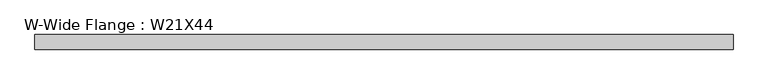
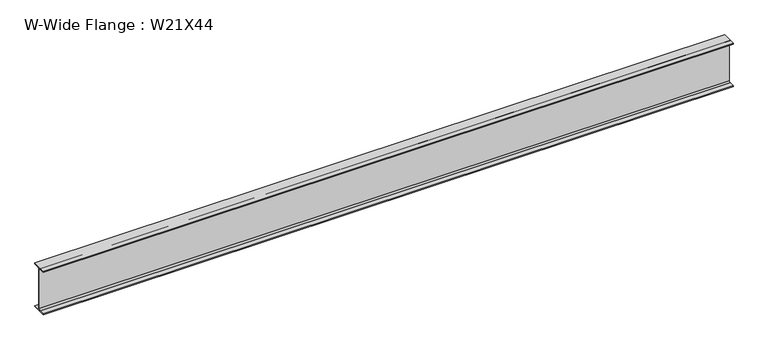
"""IFC4 building model written with IfcOpenShell, lengths in millimetres: beam geometry, W-Wide Flange : W21X44."""

from ifc_helpers import new_model, si_unit, point, frame, frame_2d, origin, place, context, project, spatial, polyline, circle_curve, trimmed, segment, composite_curve, outline, extrude, source, transform, mapped, element, save


def w_wide_flange_w21x44_d1ecdd04(model_context):
    return source(origin(), model_context, "Body", "SweptSolid", [
        extrude(outline(composite_curve([segment(polyline([(82.55, -251.46), (82.55, -262.89), (-82.55, -262.89), (-82.55, -251.46), (-21.59, -251.46)]), True, "CONTINUOUS"), segment(trimmed(circle_curve(frame_2d((-21.59, -234.315)), 17.145), [point((-21.59, -251.46))], [point((-4.445, -234.315))], True, "CARTESIAN"), True, "CONTINUOUS"), segment(polyline([(-4.445, -234.315), (-4.445, 234.315)]), True, "CONTINUOUS"), segment(trimmed(circle_curve(frame_2d((-21.59, 234.315)), 17.145), [point((-4.445, 234.315))], [point((-21.59, 251.46))], True, "CARTESIAN"), True, "CONTINUOUS"), segment(polyline([(-21.59, 251.46), (-82.55, 251.46), (-82.55, 262.89), (82.55, 262.89), (82.55, 251.46), (21.59, 251.46)]), True, "CONTINUOUS"), segment(trimmed(circle_curve(frame_2d((21.59, 234.315)), 17.145), [point((21.59, 251.46))], [point((4.445, 234.315))], True, "CARTESIAN"), True, "CONTINUOUS"), segment(polyline([(4.445, 234.315), (4.445, -234.315)]), True, "CONTINUOUS"), segment(trimmed(circle_curve(frame_2d((21.59, -234.315)), 17.145), [point((4.445, -234.315))], [point((21.59, -251.46))], True, "CARTESIAN"), True, "CONTINUOUS"), segment(polyline([(21.59, -251.46), (82.55, -251.46)]), True, "CONTINUOUS")], self_intersect=False)), frame((-3902.8161313, 0.0, 0.0), z_axis=(1.0, 0.0, 0.0), x_axis=(0.0, 1.0, 0.0)), (0.0, 0.0, 1.0), 7866.3355749),
    ])


if __name__ == "__main__":
    model = new_model("IFC4")
    model_context = context("Model", 3, world=origin())
    ifc_project = project(units=[si_unit("LENGTHUNIT", "METRE", prefix="MILLI")], contexts=[model_context])
    site = spatial("IfcSite", under=ifc_project)
    building = spatial("IfcBuilding", under=site)
    placement = place(None, origin())
    w_wide_flange_w21x44_shape = w_wide_flange_w21x44_d1ecdd04(model_context)
    element("IfcBeam", 1, ObjectType="W-Wide Flange : W21X44", at=placement, inside=building, context=model_context, shape_type="MappedRepresentation", body=[
        mapped(w_wide_flange_w21x44_shape, transform((0.0, 0.0, 0.0), x_axis=(1.0, 0.0, 0.0), y_axis=(0.0, 1.0, 0.0), z_axis=(0.0, 0.0, 1.0))),
    ])
    save(model, "model.ifc")

# Revit data of these elements
# Type "W-Wide Flange : W21X44"
#   Assembly Code = "B10"
#   W = 44
#   Length [instance default] = 1524 mm
#   bf = 165.1 mm
#   d = 525.78 mm
#   k = 28.575 mm
#   k2 = 17.145 mm
#   tf = 11.43 mm
#   tw = 8.89 mm
#   A = 0.00838708 m²
#   Structural Material [instance default] = Steel ASTM A992
# Element 1 (IfcBeam, "W-Wide Flange : W21X44")
#   Structural Material = Aluminum, Anodized Red
#   Materials on its faces: "Aluminum, Anodized Red"
# Materials
#   "Steel ASTM A992": class "Metal", colour RGB 128 0 0, transparency 0, Description = "Structural steel 50ksi", Cost = 0
#   "Aluminum, Anodized Red": class "Metal", colour RGB 120 120 120, transparency 0, Description = "Anodized aluminum, red", Cost = 0
